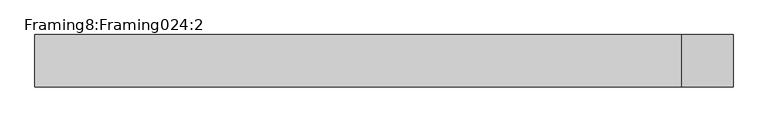
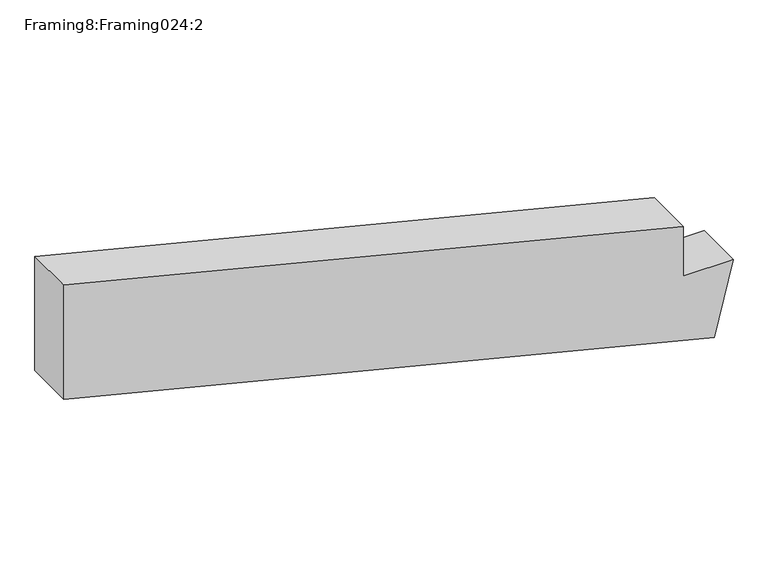
"""IFC4 building model written with IfcOpenShell, lengths in millimetres: proxy geometry, Framing8:Framing024:2 : Framing8:Framing024:286352."""

from ifc_helpers import new_model, si_unit, frame, origin, place, context, project, spatial, polyline, outline, extrude, source, transform, mapped, element, save


def framing8_framing024_2_4026ef83(model_context):
    return source(origin(), model_context, "Body", "SweptSolid", [
        extrude(outline(polyline([(110357.3362587, 15130.8894286), (110588.0006385, 15187.4083443), (110588.0006385, 15036.8413595), (110746.7842581, 15036.8413595), (111216.6873042, 13157.0903708), (110849.8516785, 13157.0903708), (110357.3362587, 15130.8894286)])), frame((0.0, -13445.349577, 0.0), z_axis=(0.0, 1.0, 0.0), x_axis=(0.0, 0.0, 1.0)), (0.0, 0.0, 1.0), 152.4),
    ])


if __name__ == "__main__":
    model = new_model("IFC4")
    model_context = context("Model", 3, world=origin())
    ifc_project = project(units=[si_unit("LENGTHUNIT", "METRE", prefix="MILLI")], contexts=[model_context])
    site = spatial("IfcSite", under=ifc_project)
    building = spatial("IfcBuilding", under=site)
    placement = place(None, origin())
    framing8_framing024_2_shape = framing8_framing024_2_4026ef83(model_context)
    element("IfcBuildingElementProxy", 1, Name="Framing8:Framing024:2 : Framing8:Framing024:286352", ObjectType="Framing8:Framing024:2 : Framing8:Framing024:286352", at=placement, inside=building, context=model_context, shape_type="MappedRepresentation", body=[
        mapped(framing8_framing024_2_shape, transform((0.0, 0.0, 0.0), x_axis=(1.0, 0.0, 0.0), y_axis=(0.0, 1.0, 0.0), z_axis=(0.0, 0.0, 1.0))),
    ])
    save(model, "model.ifc")

# Revit data of these elements
# Type "Framing8:Framing024:2 : Framing8:Framing024:286352"
#   NameOverride = "Framing8:Framing024:286352"
#   ObjectTypeOverride = "Framing8:Framing024"
#   Reference = "Framing024"
#   Category = "Generic Models"
#   Tag = "286352"
# Element 1 (IfcBuildingElementProxy, "Framing8:Framing024:2 : Framing8:Framing024:286352")
#   Materials on its faces: "WOOD FRAMING (SEE STRUCT DWGS)"
# Materials
#   "WOOD FRAMING (SEE STRUCT DWGS)": class "Unassigned", colour RGB 224 188 168, transparency 0, Cost = 0
